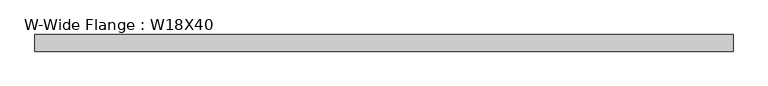
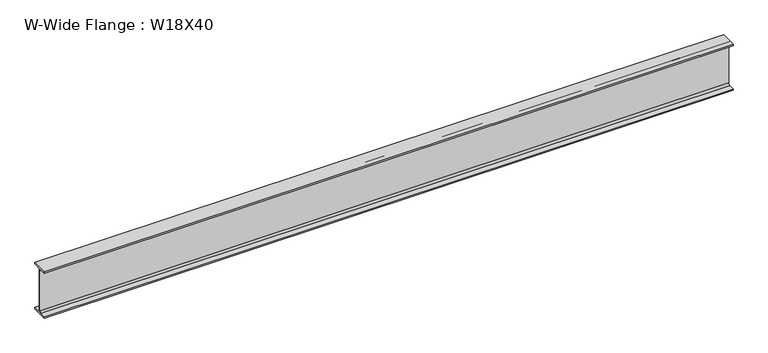
"""IFC4 building model written with IfcOpenShell, lengths in millimetres: beam geometry, W-Wide Flange : W18X40."""

from ifc_helpers import new_model, si_unit, point, frame, frame_2d, origin, place, context, project, spatial, polyline, circle_curve, trimmed, segment, composite_curve, outline, extrude, source, transform, mapped, element, save


def w_wide_flange_w18x40_a175ccdf(model_context):
    return source(origin(), model_context, "Body", "SweptSolid", [
        extrude(outline(composite_curve([segment(polyline([(76.454, -213.995), (76.454, -227.33), (-76.454, -227.33), (-76.454, -213.995), (-20.828, -213.995)]), True, "CONTINUOUS"), segment(trimmed(circle_curve(frame_2d((-20.828, -197.1675)), 16.8275), [point((-20.828, -213.995))], [point((-4.0005, -197.1675))], True, "CARTESIAN"), True, "CONTINUOUS"), segment(polyline([(-4.0005, -197.1675), (-4.0005, 197.1675)]), True, "CONTINUOUS"), segment(trimmed(circle_curve(frame_2d((-20.828, 197.1675)), 16.8275), [point((-4.0005, 197.1675))], [point((-20.828, 213.995))], True, "CARTESIAN"), True, "CONTINUOUS"), segment(polyline([(-20.828, 213.995), (-76.454, 213.995), (-76.454, 227.33), (76.454, 227.33), (76.454, 213.995), (20.828, 213.995)]), True, "CONTINUOUS"), segment(trimmed(circle_curve(frame_2d((20.828, 197.1675)), 16.8275), [point((20.828, 213.995))], [point((4.0005, 197.1675))], True, "CARTESIAN"), True, "CONTINUOUS"), segment(polyline([(4.0005, 197.1675), (4.0005, -197.1675)]), True, "CONTINUOUS"), segment(trimmed(circle_curve(frame_2d((20.828, -197.1675)), 16.8275), [point((4.0005, -197.1675))], [point((20.828, -213.995))], True, "CARTESIAN"), True, "CONTINUOUS"), segment(polyline([(20.828, -213.995), (76.454, -213.995)]), True, "CONTINUOUS")], self_intersect=False)), frame((-3206.75, 0.0, 0.0), z_axis=(1.0, 0.0, 0.0), x_axis=(0.0, 1.0, 0.0)), (0.0, 0.0, 1.0), 6418.58),
    ])


if __name__ == "__main__":
    model = new_model("IFC4")
    model_context = context("Model", 3, world=origin())
    ifc_project = project(units=[si_unit("LENGTHUNIT", "METRE", prefix="MILLI")], contexts=[model_context])
    site = spatial("IfcSite", under=ifc_project)
    building = spatial("IfcBuilding", under=site)
    placement = place(None, origin())
    w_wide_flange_w18x40_shape = w_wide_flange_w18x40_a175ccdf(model_context)
    element("IfcBeam", 1, ObjectType="W-Wide Flange : W18X40", at=placement, inside=building, context=model_context, shape_type="MappedRepresentation", body=[
        mapped(w_wide_flange_w18x40_shape, transform((0.0, 0.0, 0.0), x_axis=(1.0, 0.0, 0.0), y_axis=(0.0, 1.0, 0.0), z_axis=(0.0, 0.0, 1.0))),
    ])
    save(model, "model.ifc")

# Revit data of these elements
# Type "W-Wide Flange : W18X40"
#   Assembly Code = "B10"
#   W = 40
#   Length [instance default] = 5' - 0"
#   bf = 0' - 6.02"
#   d = 1' - 5.9"
#   k = 0' - 1 3/16"
#   k2 = 0' - 0.6625"
#   tf = 0' - 0.525"
#   tw = 0' - 0.315"
#   A = 0.0819444 SF
#   Structural Material [instance default] = Steel ASTM A992
# Element 1 (IfcBeam, "W-Wide Flange : W18X40")
#   Materials on its faces: "Steel ASTM A992"
# Materials
#   "Steel ASTM A992": class "Metal", colour RGB 199 199 199, transparency 0, Description = "Structural steel 50ksi", Cost = 0
